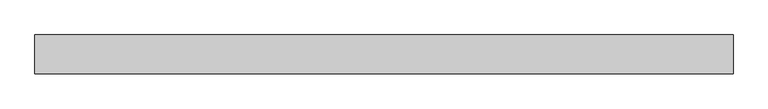
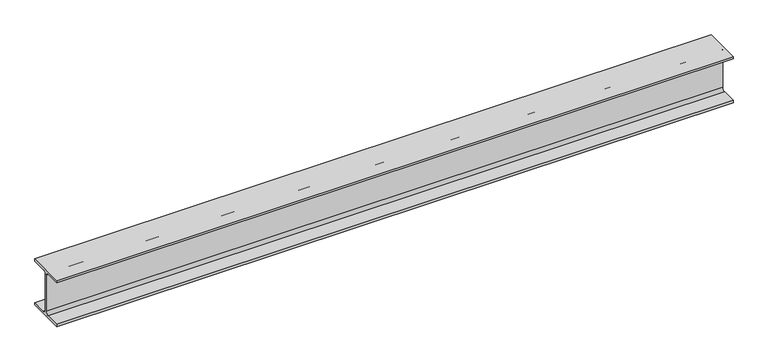
"""IFC4 building model written with IfcOpenShell, lengths in millimetres: beam geometry, 0912_Steel Framing_H-KSD3502 : H_SB_ASB_H-194x150x6x9."""

from ifc_helpers import new_model, si_unit, point, frame, frame_2d, origin, place, context, project, spatial, polyline, circle_curve, trimmed, segment, composite_curve, outline, extrude, source, transform, mapped, element, save


def beam_e749d06f(model_context):
    return source(origin(), model_context, "Body", "SweptSolid", [
        extrude(outline(composite_curve([segment(polyline([(-75.0, -88.0), (-16.0, -88.0)]), True, "CONTINUOUS"), segment(trimmed(circle_curve(frame_2d((-16.0, -75.0)), 13.0), [point((-16.0, -88.0))], [point((-3.0, -75.0))], True, "CARTESIAN"), True, "CONTINUOUS"), segment(polyline([(-3.0, -75.0), (-3.0, 75.0)]), True, "CONTINUOUS"), segment(trimmed(circle_curve(frame_2d((-16.0, 75.0)), 13.0), [point((-3.0, 75.0))], [point((-16.0, 88.0))], True, "CARTESIAN"), True, "CONTINUOUS"), segment(polyline([(-16.0, 88.0), (-75.0, 88.0), (-75.0, 97.0), (75.0, 97.0), (75.0, 88.0), (16.0, 88.0)]), True, "CONTINUOUS"), segment(trimmed(circle_curve(frame_2d((16.0, 75.0)), 13.0), [point((16.0, 88.0))], [point((3.0, 75.0))], True, "CARTESIAN"), True, "CONTINUOUS"), segment(polyline([(3.0, 75.0), (3.0, -75.0)]), True, "CONTINUOUS"), segment(trimmed(circle_curve(frame_2d((16.0, -75.0)), 13.0), [point((3.0, -75.0))], [point((16.0, -88.0))], True, "CARTESIAN"), True, "CONTINUOUS"), segment(polyline([(16.0, -88.0), (75.0, -88.0), (75.0, -97.0), (-75.0, -97.0), (-75.0, -88.0)]), True, "CONTINUOUS")], self_intersect=False)), frame((-1200.1295083, 0.0, 0.0), z_axis=(1.0, 0.0, 0.0), x_axis=(0.0, 1.0, 0.0)), (0.0, 0.0, 1.0), 2693.3121073),
    ])


if __name__ == "__main__":
    model = new_model("IFC4")
    model_context = context("Model", 3, world=origin())
    ifc_project = project(units=[si_unit("LENGTHUNIT", "METRE", prefix="MILLI")], contexts=[model_context])
    site = spatial("IfcSite", under=ifc_project)
    building = spatial("IfcBuilding", under=site)
    placement = place(None, origin())
    beam_shape = beam_e749d06f(model_context)
    element("IfcBeam", 1, ObjectType="0912_Steel Framing_H-KSD3502 : H_SB_ASB_H-194x150x6x9", at=placement, inside=building, context=model_context, shape_type="MappedRepresentation", body=[
        mapped(beam_shape, transform((0.0, 0.0, 0.0), x_axis=(1.0, 0.0, 0.0), y_axis=(0.0, 1.0, 0.0), z_axis=(0.0, 0.0, 1.0))),
    ])
    save(model, "model.ifc")

# Revit data of these elements
# Type "0912_Steel Framing_H-KSD3502 : H_SB_ASB_H-194x150x6x9"
#   H_WM Code_1 = "S01AA002-00001 | Main Steel Structure Fabrication Work | Shelter/Building | Medium Steel - Standard (90KG/M>Weight≥30KG/M) | Material: (   )"
#   H_WM Code_2 = "S03AA028-00001 | Main Steel Structure Erection Work | Shelter/Building | Medium Steel (90KG/M>Weight≥30KG/M) | Material: (   )"
#   H_WM Code_3 = "S01AA010-00001 | Main Steel Structure Fabrication Work | Shelter/Building | Steel Painting/Coating | for Non-Fireproofed Steel Surface, Surface Preparation, Primer, Second & Final Coat | Material: (   )"
#   H_Q'ty Cal Type Tag = "SB-Q2"
#   Width = 15.0 cm
#   Web Thickness = 0.6 cm
#   Web Fillet = 1.3 cm
#   Warping Constant = 43316.0 cm⁶
#   W = 0
#   Torsional Moment of Inertia = 8.622 cm⁴
#   Section Area = 39.01 cm²
#   Plastic Modulus weak axis = 104.0 cm³
#   Plastic Modulus strong axis = 309.0 cm³
#   Perimeter = 0.95 m²/m
#   Nominal Weight = 30.60 kgf/m
#   Moment of Inertia weak axis = 507.00 cm⁴
#   Moment of Inertia strong axis = 2690.00 cm⁴
#   Height = 19.4 cm
#   Flange Thickness = 0.9 cm
#   Elastic Modulus weak axis = 67.6 cm³
#   Elastic Modulus strong axis = 277.0 cm³
#   Centroid Vertical = 9.7 cm
#   Centroid Horizontal = 7.5 cm
#   Ix = 26900000
#   Length [instance default] = 1.5240 m
#   Zx = 309000
#   b = 0.1500 m
#   h = 0.1940 m
#   r = 0.0130 m
#   s = 0.0060 m
#   t = 0.0090 m
#   A = 0.003901 m²
#   Structural Material [instance default] = Steel, 45-345
#   Assembly Code = ""
# Element 1 (IfcBeam, "0912_Steel Framing_H-KSD3502 : H_SB_ASB_H-194x150x6x9")
#   Structural Material = none
# Materials
#   "Steel, 45-345": class "Metal", colour RGB 189 187 185, transparency 0, Description = "Steel 345 MPa", Cost = 0
